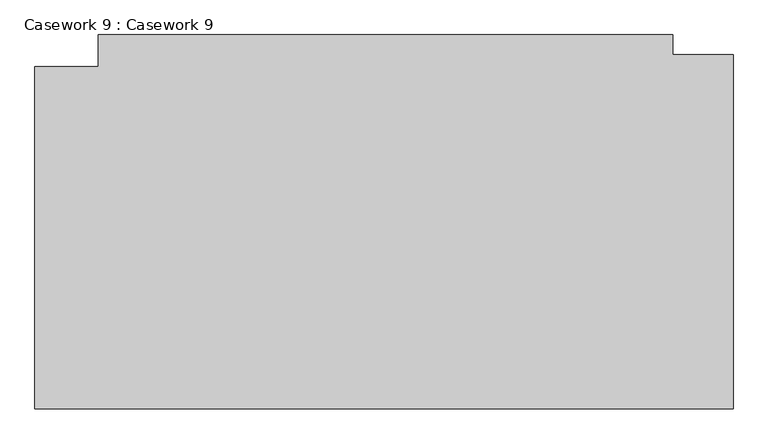
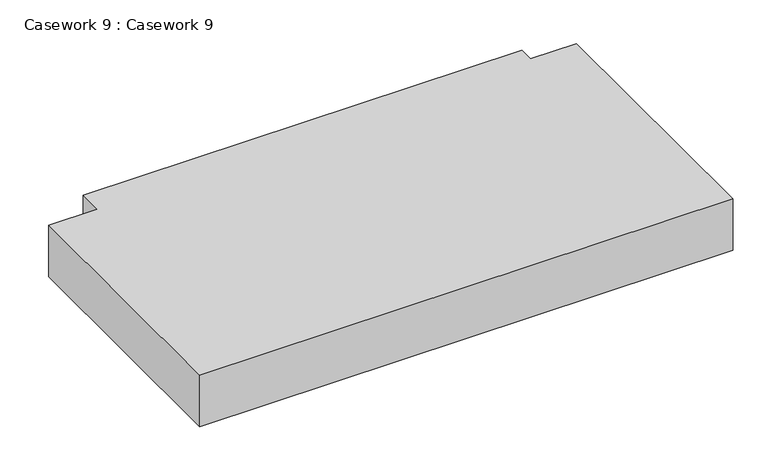
"""IFC4 building model written with IfcOpenShell, lengths in millimetres: furniture geometry, Casework 9 : Casework 9."""

from ifc_helpers import new_model, si_unit, frame, origin, place, context, project, spatial, polyline, outline, extrude, source, transform, mapped, element, save


def casework_9_casework_9_ac2b7527(model_context):
    return source(origin(), model_context, "Body", "SweptSolid", [
        extrude(outline(polyline([(-7163.5247381, -429.3850684), (-7163.5247381, -329.3850684), (-5353.5247381, -329.3850684), (-5353.5247381, -391.8265396), (-5163.5247381, -391.8265396), (-5163.5247381, -1508.8048922), (-7363.5247381, -1508.8048922), (-7363.5247381, -429.3850684), (-7163.5247381, -429.3850684)])), frame((0.0, 0.0, -225.0091615), z_axis=(0.0, 0.0, 1.0), x_axis=(1.0, 0.0, 0.0)), (0.0, 0.0, 1.0), 225.0091615),
    ])


if __name__ == "__main__":
    model = new_model("IFC4")
    model_context = context("Model", 3, world=origin())
    ifc_project = project(units=[si_unit("LENGTHUNIT", "METRE", prefix="MILLI")], contexts=[model_context])
    site = spatial("IfcSite", under=ifc_project)
    building = spatial("IfcBuilding", under=site)
    placement = place(None, origin())
    casework_9_casework_9_shape = casework_9_casework_9_ac2b7527(model_context)
    element("IfcFurniture", 1, ObjectType="Casework 9 : Casework 9", at=placement, inside=building, context=model_context, shape_type="MappedRepresentation", body=[
        mapped(casework_9_casework_9_shape, transform((0.0, 0.0, 0.0), x_axis=(1.0, 0.0, 0.0), y_axis=(0.0, 1.0, 0.0), z_axis=(0.0, 0.0, 1.0))),
    ])
    save(model, "model.ifc")

# Revit data of these elements
# Element 1 (IfcFurniture, "Casework 9 : Casework 9")
#   Materials on its faces: "Plaster"
# Materials
#   "Plaster": class "Generic", colour RGB 249 249 249, transparency 0, Description = "Plaster", Cost = 0
